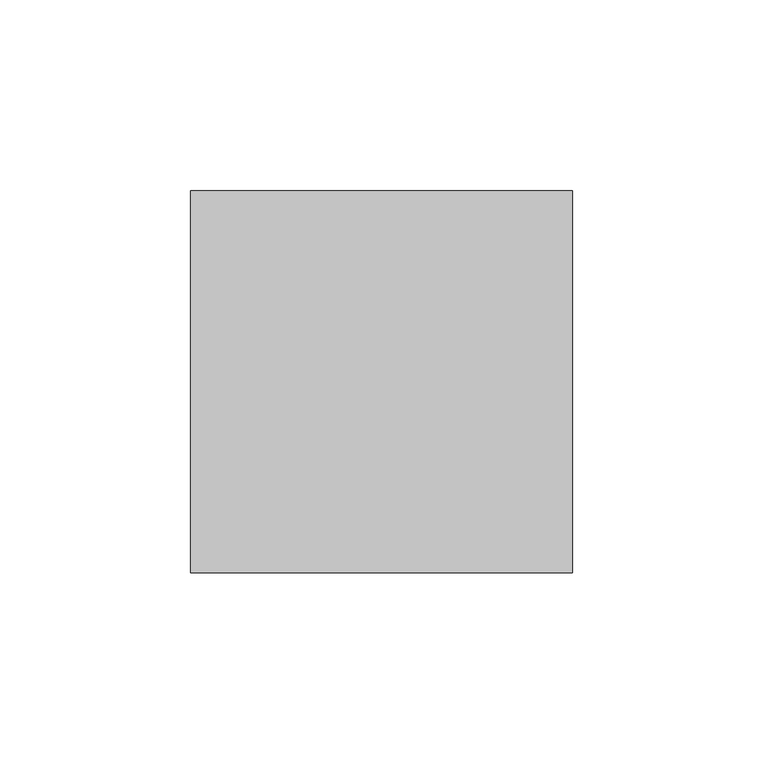
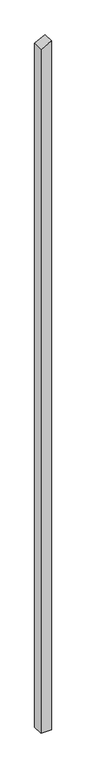
"""IFC4 building model written with IfcOpenShell, lengths in millimetres: column geometry, Holzstütze 160056 : Holzstütze 160056."""

import ifcopenshell
import ifcopenshell.guid

model = None  # the IFC model being written
_history = None  # IfcOwnerHistory: only IFC2X3 demands one
_inside = {}  # id of a spatial element -> (the spatial element, [elements in it])
_under = {}  # id of a project, library or spatial element -> (it, [spatial elements below it])
_declared = {}  # id of a project -> (the project, [libraries it declares])
_typed = {}  # id of a type object -> (the type object, [elements of that type])
_made_of = {}  # id of a material, layer set ... -> (it, [elements and type objects made of it])


def new_model(schema):
    """Start an empty IFC model of exactly this schema.

    Asked for "IFC4X3", IfcOpenShell would pick the latest addendum, in which some entities
    have other attributes; the version numbers below select the first issue.
    IFC2X3 requires an IfcOwnerHistory on every rooted entity: one is made here for all.
    """
    global model, _history
    if schema == "IFC4X3":
        model = ifcopenshell.file(schema_version=(4, 3, 0, 0))
    else:
        model = ifcopenshell.file(schema=schema)
    _inside.clear()
    _under.clear()
    _declared.clear()
    _typed.clear()
    _made_of.clear()
    _history = None
    if model.schema == "IFC2X3":
        org = make("IfcOrganization", Name="unknown")
        user = make(
            "IfcPersonAndOrganization",
            ThePerson=make("IfcPerson", FamilyName="unknown"),
            TheOrganization=org,
        )
        app = make(
            "IfcApplication",
            ApplicationDeveloper=org,
            Version="unknown",
            ApplicationFullName="unknown",
            ApplicationIdentifier="unknown",
        )
        _history = make(
            "IfcOwnerHistory",
            OwningUser=user,
            OwningApplication=app,
            ChangeAction="ADDED",
            CreationDate=0,
        )
    return model


def make(cls, **values):
    """One entity of the class cls with the attributes given. An attribute that is None is left unset."""
    return model.create_entity(
        cls, **{name: value for name, value in values.items() if value is not None}
    )


def rooted(cls, **values):
    """An entity with a GlobalId (a new one), such as an element, a storey or a relation."""
    return make(cls, GlobalId=ifcopenshell.guid.new(), OwnerHistory=_history, **values)


def si_unit(unit_type, name, prefix=None):
    """IfcSIUnit, for example si_unit("LENGTHUNIT", "METRE", prefix="MILLI")."""
    return make("IfcSIUnit", UnitType=unit_type, Prefix=prefix, Name=name)


def assignment(units):
    """IfcUnitAssignment: the units of a project."""
    return None if units is None else make("IfcUnitAssignment", Units=units)


def point(xyz):
    """IfcCartesianPoint."""
    return None if xyz is None else make("IfcCartesianPoint", Coordinates=xyz)


def direction(xyz):
    """IfcDirection."""
    return None if xyz is None else make("IfcDirection", DirectionRatios=xyz)


def frame(location, z_axis=None, x_axis=None):
    """IfcAxis2Placement3D, a coordinate frame: its origin and axes. An axis left out is left unset."""
    return make(
        "IfcAxis2Placement3D",
        Location=point(location),
        Axis=direction(z_axis),
        RefDirection=direction(x_axis),
    )


def origin():
    """The frame at (0, 0, 0) with its axes left unset."""
    return frame((0.0, 0.0, 0.0))


def place(relative_to, where):
    """IfcLocalPlacement: puts the frame where relative to a parent placement (None: the world)."""
    return make(
        "IfcLocalPlacement", PlacementRelTo=relative_to, RelativePlacement=where
    )


def context(
    kind, dimensions, precision=None, world=None, true_north=None, identifier=None
):
    """IfcGeometricRepresentationContext, for example the 3D "Model" context."""
    return make(
        "IfcGeometricRepresentationContext",
        ContextIdentifier=identifier,
        ContextType=kind,
        CoordinateSpaceDimension=dimensions,
        Precision=precision,
        WorldCoordinateSystem=world,
        TrueNorth=true_north,
    )


def project(units=None, contexts=None):
    """IfcProject with its units and contexts."""
    return rooted(
        "IfcProject",
        Name="project",
        RepresentationContexts=contexts,
        UnitsInContext=assignment(units),
    )


def spatial(cls, under=None, at=None, **own):
    """A site, building, storey or space (cls), placed at a placement, below another one or the project."""
    s = rooted(cls, ObjectPlacement=at, **own)
    if under is not None:
        _under.setdefault(under.id(), (under, []))[1].append(s)
    return s


def polyline(points):
    """IfcPolyline through the points."""
    return make("IfcPolyline", Points=[point(p) for p in points])


def outline(outer, holes=None, kind="AREA"):
    """IfcArbitraryClosedProfileDef: a profile drawn as a closed curve; with holes, ...WithVoids."""
    if holes is None:
        return make("IfcArbitraryClosedProfileDef", ProfileType=kind, OuterCurve=outer)
    return make(
        "IfcArbitraryProfileDefWithVoids",
        ProfileType=kind,
        OuterCurve=outer,
        InnerCurves=holes,
    )


def extrude(swept, where, along, depth):
    """IfcExtrudedAreaSolid: the profile swept, set in the frame where, extruded along a direction by depth."""
    return make(
        "IfcExtrudedAreaSolid",
        SweptArea=swept,
        Position=where,
        ExtrudedDirection=direction(along),
        Depth=depth,
    )


def shape(context_of_items, identifier, shape_type, items):
    """IfcShapeRepresentation: the items that make up one representation, for example the "Body"."""
    return make(
        "IfcShapeRepresentation",
        ContextOfItems=context_of_items,
        RepresentationIdentifier=identifier,
        RepresentationType=shape_type,
        Items=items,
    )


def source(mapping_origin, context_of_items, identifier, shape_type, items):
    """IfcRepresentationMap: a shape defined once, which mapped items show again and again."""
    return make(
        "IfcRepresentationMap",
        MappingOrigin=mapping_origin,
        MappedRepresentation=shape(context_of_items, identifier, shape_type, items),
    )


def transform(
    local_origin,
    x_axis=None,
    y_axis=None,
    z_axis=None,
    scale=None,
    scale2=None,
    scale3=None,
    uniform=True,
):
    """IfcCartesianTransformationOperator3D, or its non-uniform kind. x_axis, y_axis, z_axis: its Axis1, 2, 3."""
    if uniform:
        return make(
            "IfcCartesianTransformationOperator3D",
            Axis1=direction(x_axis),
            Axis2=direction(y_axis),
            LocalOrigin=point(local_origin),
            Scale=scale,
            Axis3=direction(z_axis),
        )
    return make(
        "IfcCartesianTransformationOperator3DnonUniform",
        Axis1=direction(x_axis),
        Axis2=direction(y_axis),
        LocalOrigin=point(local_origin),
        Scale=scale,
        Axis3=direction(z_axis),
        Scale2=scale2,
        Scale3=scale3,
    )


def mapped(mapping_source, mapping_target):
    """IfcMappedItem: shows the shape of a source again, moved by a transform."""
    return make(
        "IfcMappedItem", MappingSource=mapping_source, MappingTarget=mapping_target
    )


def made_of(thing, what):
    """Note that an element or type object is made of a material, layer set ...; save() writes the relation."""
    if what is not None:
        _made_of.setdefault(what.id(), (what, []))[1].append(thing)
    return thing


def element(
    cls,
    number,
    at=None,
    inside=None,
    cuts=None,
    type_object=None,
    material=None,
    context=None,
    identifier="Body",
    shape_type=None,
    held_by="IfcProductDefinitionShape",
    body=None,
    shapes=None,
    **own,
):
    """One element of the class cls, such as IfcWall. Its Tag is "e" and its number.

    at: its placement. inside: the storey or other place that contains it. cuts: it is an
    opening in that element (IfcRelVoidsElement). A single representation is given by context,
    identifier, shape_type and body (its items); several are given by shapes. held_by: the class
    of the entity that holds the representations. save() writes the other relations.
    """
    e = rooted(cls, Tag="e%d" % number, ObjectPlacement=at, **own)
    if body is not None:
        shapes = [shape(context, identifier, shape_type, body)]
    if shapes is not None:
        e.Representation = make(held_by, Representations=shapes)
    if inside is not None:
        _inside.setdefault(inside.id(), (inside, []))[1].append(e)
    if cuts is not None:
        rooted(
            "IfcRelVoidsElement", RelatingBuildingElement=cuts, RelatedOpeningElement=e
        )
    if type_object is not None:
        _typed.setdefault(type_object.id(), (type_object, []))[1].append(e)
    return made_of(e, material)


def aggregate(whole, parts):
    """IfcRelAggregates: a whole, such as a stair, and the parts it consists of."""
    return rooted("IfcRelAggregates", RelatingObject=whole, RelatedObjects=parts)


def save(model, path):
    """Write the relations noted so far, then the file.

    IfcRelAggregates (storeys below a building ...), IfcRelContainedInSpatialStructure (elements
    in a storey), IfcRelDefinesByType, IfcRelAssociatesMaterial and IfcRelDeclares: one each for
    every whole, place, type object, material and project.
    """
    for whole, parts in _under.values():
        aggregate(whole, parts)
    for where, things in _inside.values():
        rooted(
            "IfcRelContainedInSpatialStructure",
            RelatedElements=things,
            RelatingStructure=where,
        )
    for kind, things in _typed.values():
        rooted("IfcRelDefinesByType", RelatedObjects=things, RelatingType=kind)
    for what, things in _made_of.values():
        rooted("IfcRelAssociatesMaterial", RelatedObjects=things, RelatingMaterial=what)
    for by, libraries in _declared.values():
        rooted("IfcRelDeclares", RelatingContext=by, RelatedDefinitions=libraries)
    model.write(path)


def column_f815af80(model_context):
    return source(origin(), model_context, "Body", "SweptSolid", [
        extrude(outline(polyline([(-500.0, 157297.7593015), (-500.0, 157397.7593015), (6396.6643707, 157397.7593015), (6345.7118258, 157297.7593015), (-500.0, 157297.7593015)])), frame((0.0, 31941.5369795, 0.0), z_axis=(0.0, 1.0, 0.0), x_axis=(0.0, 0.0, 1.0)), (0.0, 0.0, 1.0), 100.0),
    ])


if __name__ == "__main__":
    model = new_model("IFC4")
    model_context = context("Model", 3, world=origin())
    ifc_project = project(units=[si_unit("LENGTHUNIT", "METRE", prefix="MILLI")], contexts=[model_context])
    site = spatial("IfcSite", under=ifc_project)
    building = spatial("IfcBuilding", under=site)
    placement = place(None, origin())
    column_shape = column_f815af80(model_context)
    element("IfcColumn", 1, ObjectType="Holzstütze 160056 : Holzstütze 160056", at=placement, inside=building, context=model_context, shape_type="MappedRepresentation", body=[
        mapped(column_shape, transform((0.0, 0.0, 0.0), x_axis=(1.0, 0.0, 0.0), y_axis=(0.0, 1.0, 0.0), z_axis=(0.0, 0.0, 1.0))),
    ])
    save(model, "model.ifc")

# Revit data of these elements
# Type "Holzstütze 160056 : Holzstütze 160056"
#   Abrechnungsart = "m"
#   Allright_Bauteil_ID = "0152St 0000143501"
#   Bezeichnung = "Holzstütze"
#   Codetext = "ST-HOLZ\\"
#   Gewerk = "Zimmer- und Holzbauarbeiten"
#   Material = "Holz"
#   Objektname = "Stütze"
#   NameOverride = "Holzstütze"
#   Reference = "Holzstütze"
#   Status = "NEW"
#   ThermalTransmittance = 0.0000 BTU/(h·ft²·°F)
#   Roll = 0.00°
#   Slope = 0.00°
#   2D Interaktion = yes
#   IsExternal = yes
#   LoadBearing = yes
# Element 1 (IfcColumn, "Holzstütze 160056 : Holzstütze 160056")
#   Materials on its faces: "holzschalung"
# Materials
#   "holzschalung": class "Unassigned", colour RGB 128 128 128, transparency 0
